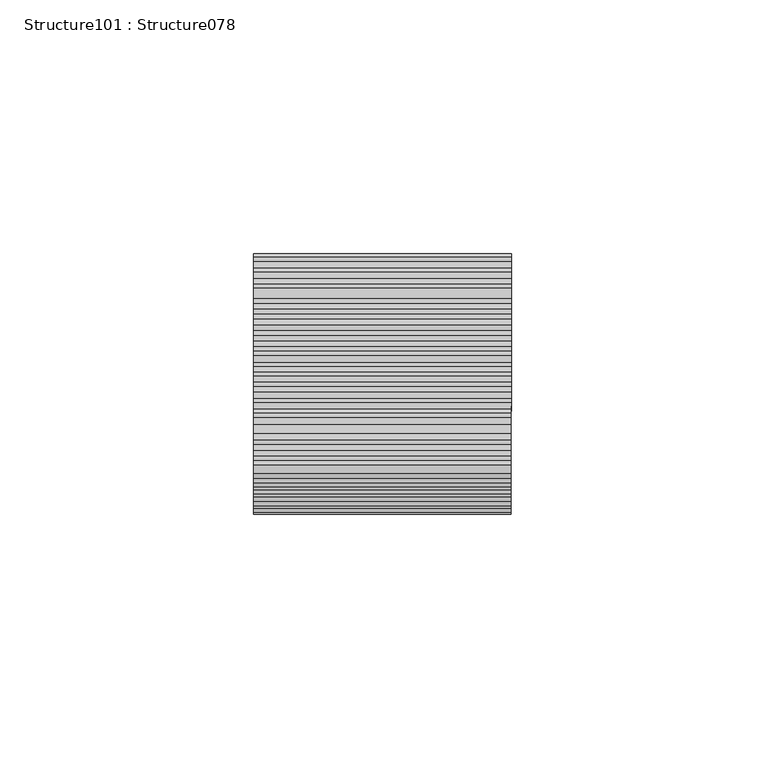
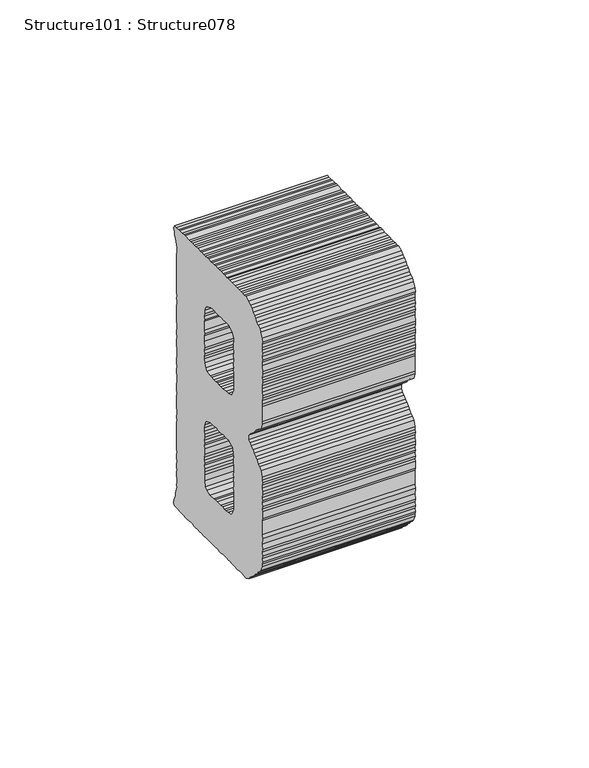
"""IFC4 building model written with IfcOpenShell, lengths in millimetres: proxy geometry, Structure101 : Structure078."""

import ifcopenshell
import ifcopenshell.guid

model = None  # the IFC model being written
_history = None  # IfcOwnerHistory: only IFC2X3 demands one
_inside = {}  # id of a spatial element -> (the spatial element, [elements in it])
_under = {}  # id of a project, library or spatial element -> (it, [spatial elements below it])
_declared = {}  # id of a project -> (the project, [libraries it declares])
_typed = {}  # id of a type object -> (the type object, [elements of that type])
_made_of = {}  # id of a material, layer set ... -> (it, [elements and type objects made of it])


def new_model(schema):
    """Start an empty IFC model of exactly this schema.

    Asked for "IFC4X3", IfcOpenShell would pick the latest addendum, in which some entities
    have other attributes; the version numbers below select the first issue.
    IFC2X3 requires an IfcOwnerHistory on every rooted entity: one is made here for all.
    """
    global model, _history
    if schema == "IFC4X3":
        model = ifcopenshell.file(schema_version=(4, 3, 0, 0))
    else:
        model = ifcopenshell.file(schema=schema)
    _inside.clear()
    _under.clear()
    _declared.clear()
    _typed.clear()
    _made_of.clear()
    _history = None
    if model.schema == "IFC2X3":
        org = make("IfcOrganization", Name="unknown")
        user = make(
            "IfcPersonAndOrganization",
            ThePerson=make("IfcPerson", FamilyName="unknown"),
            TheOrganization=org,
        )
        app = make(
            "IfcApplication",
            ApplicationDeveloper=org,
            Version="unknown",
            ApplicationFullName="unknown",
            ApplicationIdentifier="unknown",
        )
        _history = make(
            "IfcOwnerHistory",
            OwningUser=user,
            OwningApplication=app,
            ChangeAction="ADDED",
            CreationDate=0,
        )
    return model


def make(cls, **values):
    """One entity of the class cls with the attributes given. An attribute that is None is left unset."""
    return model.create_entity(
        cls, **{name: value for name, value in values.items() if value is not None}
    )


def rooted(cls, **values):
    """An entity with a GlobalId (a new one), such as an element, a storey or a relation."""
    return make(cls, GlobalId=ifcopenshell.guid.new(), OwnerHistory=_history, **values)


def si_unit(unit_type, name, prefix=None):
    """IfcSIUnit, for example si_unit("LENGTHUNIT", "METRE", prefix="MILLI")."""
    return make("IfcSIUnit", UnitType=unit_type, Prefix=prefix, Name=name)


def assignment(units):
    """IfcUnitAssignment: the units of a project."""
    return None if units is None else make("IfcUnitAssignment", Units=units)


def point(xyz):
    """IfcCartesianPoint."""
    return None if xyz is None else make("IfcCartesianPoint", Coordinates=xyz)


def direction(xyz):
    """IfcDirection."""
    return None if xyz is None else make("IfcDirection", DirectionRatios=xyz)


def frame(location, z_axis=None, x_axis=None):
    """IfcAxis2Placement3D, a coordinate frame: its origin and axes. An axis left out is left unset."""
    return make(
        "IfcAxis2Placement3D",
        Location=point(location),
        Axis=direction(z_axis),
        RefDirection=direction(x_axis),
    )


def origin():
    """The frame at (0, 0, 0) with its axes left unset."""
    return frame((0.0, 0.0, 0.0))


def place(relative_to, where):
    """IfcLocalPlacement: puts the frame where relative to a parent placement (None: the world)."""
    return make(
        "IfcLocalPlacement", PlacementRelTo=relative_to, RelativePlacement=where
    )


def context(
    kind, dimensions, precision=None, world=None, true_north=None, identifier=None
):
    """IfcGeometricRepresentationContext, for example the 3D "Model" context."""
    return make(
        "IfcGeometricRepresentationContext",
        ContextIdentifier=identifier,
        ContextType=kind,
        CoordinateSpaceDimension=dimensions,
        Precision=precision,
        WorldCoordinateSystem=world,
        TrueNorth=true_north,
    )


def project(units=None, contexts=None):
    """IfcProject with its units and contexts."""
    return rooted(
        "IfcProject",
        Name="project",
        RepresentationContexts=contexts,
        UnitsInContext=assignment(units),
    )


def spatial(cls, under=None, at=None, **own):
    """A site, building, storey or space (cls), placed at a placement, below another one or the project."""
    s = rooted(cls, ObjectPlacement=at, **own)
    if under is not None:
        _under.setdefault(under.id(), (under, []))[1].append(s)
    return s


def polyline(points):
    """IfcPolyline through the points."""
    return make("IfcPolyline", Points=[point(p) for p in points])


def outline(outer, holes=None, kind="AREA"):
    """IfcArbitraryClosedProfileDef: a profile drawn as a closed curve; with holes, ...WithVoids."""
    if holes is None:
        return make("IfcArbitraryClosedProfileDef", ProfileType=kind, OuterCurve=outer)
    return make(
        "IfcArbitraryProfileDefWithVoids",
        ProfileType=kind,
        OuterCurve=outer,
        InnerCurves=holes,
    )


def extrude(swept, where, along, depth):
    """IfcExtrudedAreaSolid: the profile swept, set in the frame where, extruded along a direction by depth."""
    return make(
        "IfcExtrudedAreaSolid",
        SweptArea=swept,
        Position=where,
        ExtrudedDirection=direction(along),
        Depth=depth,
    )


def shape(context_of_items, identifier, shape_type, items):
    """IfcShapeRepresentation: the items that make up one representation, for example the "Body"."""
    return make(
        "IfcShapeRepresentation",
        ContextOfItems=context_of_items,
        RepresentationIdentifier=identifier,
        RepresentationType=shape_type,
        Items=items,
    )


def source(mapping_origin, context_of_items, identifier, shape_type, items):
    """IfcRepresentationMap: a shape defined once, which mapped items show again and again."""
    return make(
        "IfcRepresentationMap",
        MappingOrigin=mapping_origin,
        MappedRepresentation=shape(context_of_items, identifier, shape_type, items),
    )


def transform(
    local_origin,
    x_axis=None,
    y_axis=None,
    z_axis=None,
    scale=None,
    scale2=None,
    scale3=None,
    uniform=True,
):
    """IfcCartesianTransformationOperator3D, or its non-uniform kind. x_axis, y_axis, z_axis: its Axis1, 2, 3."""
    if uniform:
        return make(
            "IfcCartesianTransformationOperator3D",
            Axis1=direction(x_axis),
            Axis2=direction(y_axis),
            LocalOrigin=point(local_origin),
            Scale=scale,
            Axis3=direction(z_axis),
        )
    return make(
        "IfcCartesianTransformationOperator3DnonUniform",
        Axis1=direction(x_axis),
        Axis2=direction(y_axis),
        LocalOrigin=point(local_origin),
        Scale=scale,
        Axis3=direction(z_axis),
        Scale2=scale2,
        Scale3=scale3,
    )


def mapped(mapping_source, mapping_target):
    """IfcMappedItem: shows the shape of a source again, moved by a transform."""
    return make(
        "IfcMappedItem", MappingSource=mapping_source, MappingTarget=mapping_target
    )


def made_of(thing, what):
    """Note that an element or type object is made of a material, layer set ...; save() writes the relation."""
    if what is not None:
        _made_of.setdefault(what.id(), (what, []))[1].append(thing)
    return thing


def element(
    cls,
    number,
    at=None,
    inside=None,
    cuts=None,
    type_object=None,
    material=None,
    context=None,
    identifier="Body",
    shape_type=None,
    held_by="IfcProductDefinitionShape",
    body=None,
    shapes=None,
    **own,
):
    """One element of the class cls, such as IfcWall. Its Tag is "e" and its number.

    at: its placement. inside: the storey or other place that contains it. cuts: it is an
    opening in that element (IfcRelVoidsElement). A single representation is given by context,
    identifier, shape_type and body (its items); several are given by shapes. held_by: the class
    of the entity that holds the representations. save() writes the other relations.
    """
    e = rooted(cls, Tag="e%d" % number, ObjectPlacement=at, **own)
    if body is not None:
        shapes = [shape(context, identifier, shape_type, body)]
    if shapes is not None:
        e.Representation = make(held_by, Representations=shapes)
    if inside is not None:
        _inside.setdefault(inside.id(), (inside, []))[1].append(e)
    if cuts is not None:
        rooted(
            "IfcRelVoidsElement", RelatingBuildingElement=cuts, RelatedOpeningElement=e
        )
    if type_object is not None:
        _typed.setdefault(type_object.id(), (type_object, []))[1].append(e)
    return made_of(e, material)


def aggregate(whole, parts):
    """IfcRelAggregates: a whole, such as a stair, and the parts it consists of."""
    return rooted("IfcRelAggregates", RelatingObject=whole, RelatedObjects=parts)


def save(model, path):
    """Write the relations noted so far, then the file.

    IfcRelAggregates (storeys below a building ...), IfcRelContainedInSpatialStructure (elements
    in a storey), IfcRelDefinesByType, IfcRelAssociatesMaterial and IfcRelDeclares: one each for
    every whole, place, type object, material and project.
    """
    for whole, parts in _under.values():
        aggregate(whole, parts)
    for where, things in _inside.values():
        rooted(
            "IfcRelContainedInSpatialStructure",
            RelatedElements=things,
            RelatingStructure=where,
        )
    for kind, things in _typed.values():
        rooted("IfcRelDefinesByType", RelatedObjects=things, RelatingType=kind)
    for what, things in _made_of.values():
        rooted("IfcRelAssociatesMaterial", RelatedObjects=things, RelatingMaterial=what)
    for by, libraries in _declared.values():
        rooted("IfcRelDeclares", RelatingContext=by, RelatedDefinitions=libraries)
    model.write(path)


def structure101_structure078_d191271b(model_context):
    return source(origin(), model_context, "Body", "SweptSolid", [
        extrude(outline(polyline([(1.021083, 1e-07), (2.2021055, -0.2015733), (3.2126148, -0.2038769), (4.2007986, -0.5720119), (5.0440335, -0.3728197), (6.4302813, -0.4104967), (7.423184, -0.59436), (8.4067138, -0.9663588), (9.4346593, -0.7807699), (11.2137025, -1.5004972), (11.9445592, -2.5830858), (12.504629, -3.4666321), (13.1675904, -4.2652239), (13.7720782, -4.7844835), (14.5344188, -5.5005744), (15.1832292, -6.4843315), (16.5089247, -8.0812413), (17.0724037, -8.9688942), (17.7699069, -9.3979872), (18.3160529, -10.4669725), (19.5597022, -11.9650508), (20.5099353, -12.6985779), (21.0906231, -13.3980644), (21.6335873, -14.4632169), (22.5838204, -15.196744), (22.9830828, -15.8798998), (23.909516, -16.7936539), (24.3090056, -17.4770835), (24.9717398, -18.2754015), (25.6204468, -19.2657186), (26.9840933, -20.4972364), (27.4450112, -21.4635573), (28.3918351, -22.1929778), (29.0406456, -23.1767349), (29.8029862, -23.8928259), (30.4657203, -24.6911439), (30.8477738, -25.562466), (31.4284616, -26.2619525), (32.2793155, -27.0779806), (32.956428, -27.6914071), (33.6050111, -28.6748904), (34.0832619, -29.4598788), (37.4860244, -33.5587876), (37.0402391, -34.4361665), (36.053481, -35.081919), (34.8237658, -35.4350096), (33.8746847, -35.7155973), (33.0899701, -36.1936208), (30.8714565, -37.1872209), (30.4416351, -37.8844038), (29.4752212, -38.3463238), (28.5753339, -39.093377), (27.943469, -39.9582889), (26.9642731, -40.6042378), (26.1749043, -41.086125), (25.560646, -41.7694772), (24.7628754, -42.4317568), (23.8787817, -42.9922811), (23.0462422, -44.0237856), (22.2443651, -44.6894743), (21.3773304, -45.0688935), (20.7410852, -45.9374418), (19.7618892, -46.5833907), (18.9643925, -47.2454431), (18.4449625, -47.843598), (17.3631022, -48.574775), (16.8480526, -49.1692936), (15.8441321, -50.0027113), (14.9629464, -50.5672957), (14.3498866, -51.2431787), (13.3632988, -51.895264), (12.6809748, -52.2882866), (12.0460983, -53.1556985), (10.8822952, -53.7814839), (10.1828087, -54.3621717), (9.3662331, -55.2134803), (8.0493064, -56.4736875), (7.0654564, -57.1235), (6.2679596, -57.7855524), (5.483245, -58.2635758), (4.7487158, -59.2137159), (4.0536096, -59.7907673), (3.1680435, -60.3589881), (2.182928, -61.003377), (0.6840284, -62.2477081), (-0.0296091, -63.0135611), (-1.0321607, -63.8458425), (-1.8138639, -64.321366), (-2.5486669, -65.2717332), (-3.4325903, -65.8385904), (-5.0148017, -66.9786662), (-6.7110906, -68.3868626), (-7.2303503, -68.9913504), (-8.9266392, -70.3995468), (-9.814292, -70.9630257), (-10.4458832, -71.8277104), (-11.3256999, -72.3911583), (-12.3124581, -73.0369109), (-13.1113237, -73.7000995), (-13.7285935, -74.3859518), (-14.5436968, -75.2295638), (-16.1447133, -76.5586685), (-16.8241293, -76.9557512), (-17.7418969, -77.8845913), (-19.3078706, -78.8442438), (-20.1447904, -79.8793847), (-21.0088137, -80.2563039), (-21.6230721, -80.9396561), (-22.5408397, -81.8684963), (-23.2243623, -82.2689881), (-24.0391918, -83.1123728), (-25.7384923, -84.5230693), (-26.5244054, -85.0085619), (-28.2190518, -86.4153947), (-28.8414199, -87.0990051), (-29.820342, -87.7447267), (-30.339772, -88.3428816), (-32.0346921, -89.7499417), (-32.9061071, -90.1329972), (-33.9056473, -90.9627786), (-35.1517706, -92.5110427), (-35.4995922, -93.3075582), (-35.9701023, -94.3724059), (-36.6871954, -95.1346535), (-37.1533249, -96.1958648), (-38.4729224, -96.4501547), (-38.9498043, -95.6640299), (-39.7798129, -94.6642159), (-40.3827149, -94.1496518), (-41.2129508, -93.149564), (-41.9736953, -92.4326105), (-42.4725641, -91.8316818), (-43.5962161, -90.0670428), (-44.2623594, -89.2646182), (-45.127137, -88.6340292), (-45.69527, -87.7502401), (-46.2759578, -87.0507536), (-47.1189759, -86.2346947), (-47.6651219, -85.1657095), (-48.349843, -84.5525875), (-48.9908175, -83.5687996), (-49.760994, -82.8527395), (-50.3416819, -82.153253), (-51.0206073, -81.5348572), (-51.6487997, -80.3670404), (-52.2482926, -79.8565828), (-53.0944924, -79.0366912), (-53.5931339, -78.4360362), (-54.2433132, -77.4534155), (-54.8240011, -76.753929), (-55.5849728, -76.0367017), (-56.3171984, -74.9552495), (-56.9106683, -74.4397918), (-57.5388607, -73.271975), (-58.239773, -72.8387754), (-58.8204608, -72.1392889), (-59.5558684, -71.0540038), (-60.7142895, -69.6585898), (-61.6425356, -68.7398667), (-62.02118, -67.8726511), (-62.8702209, -67.0615923), (-63.5363642, -66.2591676), (-64.0130188, -65.4733166), (-64.7959774, -64.9412854), (-65.2754266, -63.1426832), (-65.1566279, -61.8625089), (-65.3378366, -60.8309269), (-65.1326112, -59.6459477), (-64.9488822, -58.6517692), (-65.14747, -57.8020207), (-64.6801988, -56.7393993), (-64.7587894, -55.6230902), (-64.8422616, -54.5103711), (-64.4770501, -53.5264642), (-63.7711534, -51.9318579), (-62.9418992, -50.9030807), (-62.0721267, -50.5213888), (-61.1749771, -49.7766083), (-60.6555472, -49.1784534), (-59.9383507, -48.4096457), (-58.8565939, -47.6850288), (-58.1440515, -46.9200848), (-57.3549565, -46.438425), (-56.3757606, -45.7924761), (-54.9420186, -44.2618755), (-54.2425321, -43.6811876), (-53.255774, -43.0354352), (-52.6412418, -42.3518556), (-51.9417553, -41.7711678), (-50.8773312, -41.2278833), (-50.0795608, -40.5656037), (-49.2600771, -39.7183553), (-48.5431544, -38.9497749), (-47.7442889, -38.2865862), (-46.9593004, -37.8083354), (-46.0624246, -37.0637823), (-45.2806179, -36.5816987), (-41.1814354, -33.1787089), (-40.5607101, -32.4964622), (-38.74618, -31.8317599), (-37.5862766, -32.2173464), (-36.5850368, -32.4012254), (-35.5919637, -32.5914215), (-34.390597, -32.6091624), (-33.2774233, -32.5262378), (-32.4608942, -32.6965133), (-31.4636112, -32.8767403), (-30.200372, -33.1834779), (-28.9848077, -33.0155526), (-27.8858884, -32.1032704), (-27.7022059, -31.1095927), (-27.7983566, -30.1743424), (-27.6825695, -28.8966681), (-27.6793412, -27.8789169), (-27.4753144, -26.7014069), (-27.579301, -25.7661874), (-27.2756213, -24.5059494), (-27.3720459, -23.5709262), (-27.3509837, -22.3718891), (-26.1809407, -20.7258525), (-25.3820751, -20.0626638), (-24.9519798, -19.3652536), (-24.0648746, -18.8022292), (-23.2671041, -18.1399497), (-22.5504552, -17.3715966), (-21.6516629, -16.6254525), (-20.768938, -16.0660645), (-20.0520153, -15.2974842), (-19.1882659, -14.9207923), (-18.4540103, -13.9708795), (-17.5666313, -13.4076279), (-17.0547636, -12.8092766), (-15.2530726, -11.3135792), (-14.3893231, -10.9368874), (-10.5912893, -7.7839001), (-9.7543694, -6.7487591), (-7.9904589, -5.6247868), (-6.8567706, -4.3432797), (-5.9737719, -3.7836644), (-5.0594599, -2.8512187), (-4.0930461, -2.3892987), (-3.4581696, -1.5218867), (-2.5914087, -1.1426948), (-1.8919222, -0.562007), (0.0, 0.0), (1.021083, 1e-07)]), holes=[polyline([(-32.0402527, -47.0360163), (-32.924894, -47.5969952), (-33.9244342, -48.4267765), (-35.3234072, -49.5881522), (-36.125558, -50.2540682), (-36.8565748, -51.2017547), (-37.6195298, -51.4943083), (-38.2558215, -52.3633576), (-40.0199594, -53.4870562), (-40.6546086, -54.354742), (-41.6340317, -55.0004171), (-43.0533955, -56.3461263), (-43.7531558, -56.9270414), (-44.6342949, -57.4911247), (-45.5358249, -58.2395416), (-46.2341594, -59.8343443), (-45.8262315, -62.3600944), (-45.2421345, -63.0636874), (-44.4811163, -63.7804137), (-43.6367295, -64.5953362), (-43.2502957, -65.4630219), (-42.2255785, -66.2951842), (-40.8967011, -67.8959269), (-40.5957227, -68.6606745), (-39.9327613, -69.4592663), (-39.1715158, -70.1762663), (-37.4052548, -71.0800226), (-36.4079716, -71.2602495), (-34.7938994, -70.7679716), (-34.0802619, -70.0021186), (-33.1149897, -69.5416086), (-32.4806143, -68.6741502), (-31.7157429, -68.3800057), (-29.3125756, -66.384985), (-28.680938, -65.5197994), (-27.8183301, -65.1445176), (-26.3166927, -63.8979138), (-24.8831781, -62.3670394), (-23.8185267, -61.8240286), (-23.2818878, -61.0377074), (-22.2175102, -60.4949239), (-21.6160339, -59.9956005), (-20.7837217, -58.9638222), (-20.097942, -57.5533222), (-19.9142595, -56.5596447), (-20.6763263, -54.8222435), (-21.2540595, -54.126316), (-21.9031438, -53.1427863), (-22.5658779, -52.3444682), (-23.2490802, -51.7231487), (-23.7306627, -50.9413887), (-24.6568221, -50.0274073), (-25.1418137, -49.2415407), (-26.6692789, -47.8121325), (-27.4174685, -46.9108763), (-28.9917305, -46.0211471), (-31.4232567, -46.3503914), (-32.0402527, -47.0360163)]), polyline([(-14.9308199, -34.6886598), (-14.5537612, -36.5722629), (-13.9525018, -37.0881907), (-13.2897677, -37.8865088), (-12.6471505, -38.8689331), (-11.960663, -39.4875252), (-11.2158825, -40.3846748), (-10.4549109, -41.1019022), (-10.0712148, -41.9718606), (-9.0439872, -42.8014765), (-7.7969288, -44.3036613), (-6.3179394, -45.2724822), (-5.5048194, -45.4386511), (-3.8045942, -45.0417957), (-2.9231812, -44.4774851), (-2.0230202, -43.7302046), (-1.3886449, -42.8627462), (-0.691896, -42.2843311), (0.4751459, -41.6563195), (1.0071307, -40.8738619), (1.8743927, -40.4947165), (2.508768, -39.6272581), (4.0076677, -38.382927), (5.0766993, -37.8362799), (5.8741961, -37.1742275), (6.4886713, -36.4967071), (7.2748117, -36.0114882), (7.9050804, -35.147439), (8.7069576, -34.4817502), (9.6893353, -33.8396341), (11.2906255, -32.5103022), (12.2570394, -31.0272991), (12.3586757, -29.9347901), (11.6991698, -28.1187208), (10.3700651, -26.5177043), (9.5052875, -25.8871152), (8.9418086, -24.9994625), (7.6981594, -23.5013842), (6.8473055, -22.6853561), (6.4718429, -21.8219734), (5.7063206, -21.1020497), (4.7734203, -20.1871901), (3.4790381, -19.2385327), (2.6485853, -19.2536962), (0.7507435, -19.8141431), (-0.7465135, -21.0571105), (-1.7332716, -21.702863), (-2.4501943, -22.4714434), (-3.2493337, -23.1348594), (-4.1364389, -23.6978837), (-4.7680765, -24.5630693), (-5.5454563, -25.0410155), (-6.5322144, -25.6867679), (-6.9648201, -26.3867246), (-8.031114, -26.9310991), (-8.5661103, -27.7160566), (-9.5327514, -28.1777029), (-10.3474106, -29.0274205), (-11.0297346, -29.4204431), (-11.6657526, -30.2892651), (-12.6655666, -31.1192737), (-13.630565, -31.5795563), (-14.0645396, -32.2806494), (-15.1292374, -33.8452442), (-14.9308199, -34.6886598)])]), frame((-56111.7599543, 290753.2996796, -367.9309464), z_axis=(-0.9999998917542983, 0.00046528635450596156, 0.0), x_axis=(0.00029719872703022485, 0.6387436295479682, -0.7694195782437595)), (0.0, 0.0, 1.0), 50.8),
    ])


if __name__ == "__main__":
    model = new_model("IFC4")
    model_context = context("Model", 3, world=origin())
    ifc_project = project(units=[si_unit("LENGTHUNIT", "METRE", prefix="MILLI")], contexts=[model_context])
    site = spatial("IfcSite", under=ifc_project)
    building = spatial("IfcBuilding", under=site)
    placement = place(None, origin())
    structure101_structure078_shape = structure101_structure078_d191271b(model_context)
    element("IfcBuildingElementProxy", 1, Name="Structure101 : Structure078", ObjectType="Structure101 : Structure078", at=placement, inside=building, context=model_context, shape_type="MappedRepresentation", body=[
        mapped(structure101_structure078_shape, transform((0.0, 0.0, 0.0), x_axis=(1.0, 0.0, 0.0), y_axis=(0.0, 1.0, 0.0), z_axis=(0.0, 0.0, 1.0))),
    ])
    save(model, "model.ifc")

# Revit data of these elements
# Type "Structure101 : Structure078"
#   NameOverride = "Structure078"
# Element 1 (IfcBuildingElementProxy, "Structure101 : Structure078")
#   Materials on its faces: "BRUSHED ALUMINUM LETTERING"
# Materials
#   "BRUSHED ALUMINUM LETTERING": class "Unassigned", colour RGB 169 181 186, transparency 0, Cost = 0
